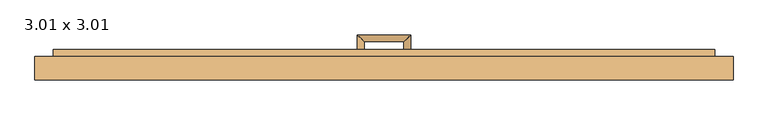
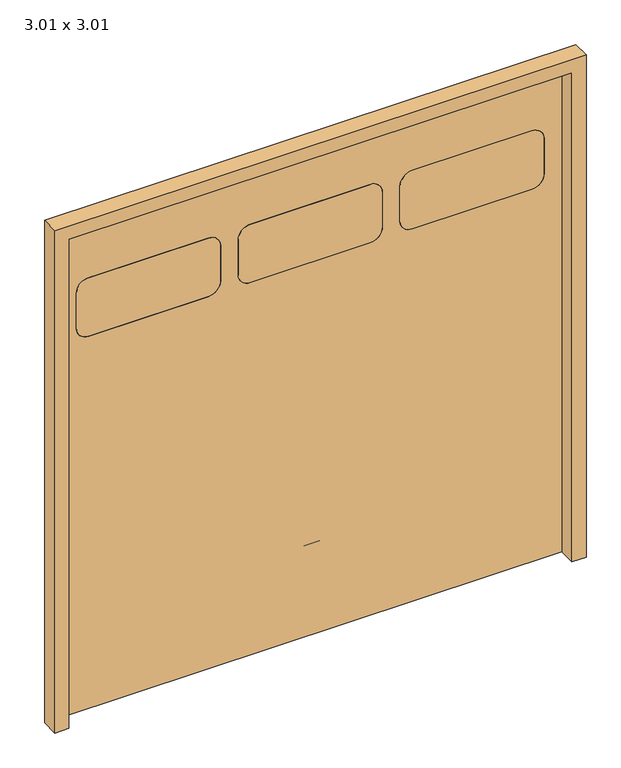
"""IFC4 building model written with IfcOpenShell, lengths in millimetres: door geometry, Garagentor : 3.01 x 3.01."""

from ifc_helpers import new_model, si_unit, point, frame, frame_2d, origin, place, context, project, spatial, polyline, circle_curve, ellipse_curve, trimmed, segment, composite_curve, outline, extrude, source, transform, mapped, element, save
from ifc_brep_helpers import plane_surface, cylinder_surface, advanced_brep


def door_3_01_x_3_01_f5100d20(model_context):
    return source(origin(), model_context, "Body", "SolidModel", [
        extrude(outline(composite_curve([segment(polyline([(2580.0, 1255.0), (2580.0, 578.3333333)]), True, "CONTINUOUS"), segment(trimmed(circle_curve(frame_2d((2510.0, 578.3333333)), 70.0), [point((2580.0, 578.3333333))], [point((2510.0, 508.3333333))], False, "CARTESIAN"), True, "CONTINUOUS"), segment(polyline([(2510.0, 508.3333333), (2300.0, 508.3333333)]), True, "CONTINUOUS"), segment(trimmed(circle_curve(frame_2d((2300.0, 578.3333333)), 70.0), [point((2300.0, 508.3333333))], [point((2230.0, 578.3333333))], False, "CARTESIAN"), True, "CONTINUOUS"), segment(polyline([(2230.0, 578.3333333), (2230.0, 1255.0)]), True, "CONTINUOUS"), segment(trimmed(circle_curve(frame_2d((2300.0, 1255.0)), 70.0), [point((2230.0, 1255.0))], [point((2300.0, 1325.0))], False, "CARTESIAN"), True, "CONTINUOUS"), segment(polyline([(2300.0, 1325.0), (2510.0, 1325.0)]), True, "CONTINUOUS"), segment(trimmed(circle_curve(frame_2d((2510.0, 1255.0)), 70.0), [point((2510.0, 1325.0))], [point((2580.0, 1255.0))], False, "CARTESIAN"), True, "CONTINUOUS")], self_intersect=False)), frame((0.0, -138.4216391, 0.0), z_axis=(0.0, 1.0, 0.0), x_axis=(0.0, 0.0, 1.0)), (0.0, 0.0, 1.0), 30.0),
        extrude(outline(composite_curve([segment(trimmed(circle_curve(frame_2d((2510.0, 338.3333333)), 70.0), [point((2510.0, 408.3333333))], [point((2580.0, 338.3333333))], False, "CARTESIAN"), True, "CONTINUOUS"), segment(polyline([(2580.0, 338.3333333), (2580.0, -338.3333333)]), True, "CONTINUOUS"), segment(trimmed(circle_curve(frame_2d((2510.0, -338.3333333)), 70.0), [point((2580.0, -338.3333333))], [point((2510.0, -408.3333333))], False, "CARTESIAN"), True, "CONTINUOUS"), segment(polyline([(2510.0, -408.3333333), (2300.0, -408.3333333)]), True, "CONTINUOUS"), segment(trimmed(circle_curve(frame_2d((2300.0, -338.3333333)), 70.0), [point((2300.0, -408.3333333))], [point((2230.0, -338.3333333))], False, "CARTESIAN"), True, "CONTINUOUS"), segment(polyline([(2230.0, -338.3333333), (2230.0, 338.3333333)]), True, "CONTINUOUS"), segment(trimmed(circle_curve(frame_2d((2300.0, 338.3333333)), 70.0), [point((2230.0, 338.3333333))], [point((2300.0, 408.3333333))], False, "CARTESIAN"), True, "CONTINUOUS"), segment(polyline([(2300.0, 408.3333333), (2510.0, 408.3333333)]), True, "CONTINUOUS")], self_intersect=False)), frame((0.0, -138.4216391, 0.0), z_axis=(0.0, 1.0, 0.0), x_axis=(0.0, 0.0, 1.0)), (0.0, 0.0, 1.0), 30.0),
        extrude(outline(composite_curve([segment(trimmed(circle_curve(frame_2d((2510.0, -578.3333333)), 70.0), [point((2510.0, -508.3333333))], [point((2580.0, -578.3333333))], False, "CARTESIAN"), True, "CONTINUOUS"), segment(polyline([(2580.0, -578.3333333), (2580.0, -1255.0)]), True, "CONTINUOUS"), segment(trimmed(circle_curve(frame_2d((2510.0, -1255.0)), 70.0), [point((2580.0, -1255.0))], [point((2510.0, -1325.0))], False, "CARTESIAN"), True, "CONTINUOUS"), segment(polyline([(2510.0, -1325.0), (2300.0, -1325.0)]), True, "CONTINUOUS"), segment(trimmed(circle_curve(frame_2d((2300.0, -1255.0)), 70.0), [point((2300.0, -1325.0))], [point((2230.0, -1255.0))], False, "CARTESIAN"), True, "CONTINUOUS"), segment(polyline([(2230.0, -1255.0), (2230.0, -578.3333333)]), True, "CONTINUOUS"), segment(trimmed(circle_curve(frame_2d((2300.0, -578.3333333)), 70.0), [point((2230.0, -578.3333333))], [point((2300.0, -508.3333333))], False, "CARTESIAN"), True, "CONTINUOUS"), segment(polyline([(2300.0, -508.3333333), (2510.0, -508.3333333)]), True, "CONTINUOUS")], self_intersect=False)), frame((0.0, -138.4216391, 0.0), z_axis=(0.0, 1.0, 0.0), x_axis=(0.0, 0.0, 1.0)), (0.0, 0.0, 1.0), 30.0),
        extrude(outline(polyline([(0.0, -1425.0), (0.0, 1425.0), (2930.0, 1425.0), (2930.0, -1425.0), (0.0, -1425.0)]), holes=[composite_curve([segment(polyline([(2580.0, 578.3333333), (2580.0, 1255.0)]), True, "CONTINUOUS"), segment(trimmed(circle_curve(frame_2d((2510.0, 1255.0)), 70.0), [point((2580.0, 1255.0))], [point((2510.0, 1325.0))], True, "CARTESIAN"), True, "CONTINUOUS"), segment(polyline([(2510.0, 1325.0), (2300.0, 1325.0)]), True, "CONTINUOUS"), segment(trimmed(circle_curve(frame_2d((2300.0, 1255.0)), 70.0), [point((2300.0, 1325.0))], [point((2230.0, 1255.0))], True, "CARTESIAN"), True, "CONTINUOUS"), segment(polyline([(2230.0, 1255.0), (2230.0, 578.3333333)]), True, "CONTINUOUS"), segment(trimmed(circle_curve(frame_2d((2300.0, 578.3333333)), 70.0), [point((2230.0, 578.3333333))], [point((2300.0, 508.3333333))], True, "CARTESIAN"), True, "CONTINUOUS"), segment(polyline([(2300.0, 508.3333333), (2510.0, 508.3333333)]), True, "CONTINUOUS"), segment(trimmed(circle_curve(frame_2d((2510.0, 578.3333333)), 70.0), [point((2510.0, 508.3333333))], [point((2580.0, 578.3333333))], True, "CARTESIAN"), True, "CONTINUOUS")], self_intersect=False), composite_curve([segment(polyline([(2580.0, -338.3333333), (2580.0, 338.3333333)]), True, "CONTINUOUS"), segment(trimmed(circle_curve(frame_2d((2510.0, 338.3333333)), 70.0), [point((2580.0, 338.3333333))], [point((2510.0, 408.3333333))], True, "CARTESIAN"), True, "CONTINUOUS"), segment(polyline([(2510.0, 408.3333333), (2300.0, 408.3333333)]), True, "CONTINUOUS"), segment(trimmed(circle_curve(frame_2d((2300.0, 338.3333333)), 70.0), [point((2300.0, 408.3333333))], [point((2230.0, 338.3333333))], True, "CARTESIAN"), True, "CONTINUOUS"), segment(polyline([(2230.0, 338.3333333), (2230.0, -338.3333333)]), True, "CONTINUOUS"), segment(trimmed(circle_curve(frame_2d((2300.0, -338.3333333)), 70.0), [point((2230.0, -338.3333333))], [point((2300.0, -408.3333333))], True, "CARTESIAN"), True, "CONTINUOUS"), segment(polyline([(2300.0, -408.3333333), (2510.0, -408.3333333)]), True, "CONTINUOUS"), segment(trimmed(circle_curve(frame_2d((2510.0, -338.3333333)), 70.0), [point((2510.0, -408.3333333))], [point((2580.0, -338.3333333))], True, "CARTESIAN"), True, "CONTINUOUS")], self_intersect=False), composite_curve([segment(polyline([(2580.0, -1255.0), (2580.0, -578.3333333)]), True, "CONTINUOUS"), segment(trimmed(circle_curve(frame_2d((2510.0, -578.3333333)), 70.0), [point((2580.0, -578.3333333))], [point((2510.0, -508.3333333))], True, "CARTESIAN"), True, "CONTINUOUS"), segment(polyline([(2510.0, -508.3333333), (2300.0, -508.3333333)]), True, "CONTINUOUS"), segment(trimmed(circle_curve(frame_2d((2300.0, -578.3333333)), 70.0), [point((2300.0, -508.3333333))], [point((2230.0, -578.3333333))], True, "CARTESIAN"), True, "CONTINUOUS"), segment(polyline([(2230.0, -578.3333333), (2230.0, -1255.0)]), True, "CONTINUOUS"), segment(trimmed(circle_curve(frame_2d((2300.0, -1255.0)), 70.0), [point((2230.0, -1255.0))], [point((2300.0, -1325.0))], True, "CARTESIAN"), True, "CONTINUOUS"), segment(polyline([(2300.0, -1325.0), (2510.0, -1325.0)]), True, "CONTINUOUS"), segment(trimmed(circle_curve(frame_2d((2510.0, -1255.0)), 70.0), [point((2510.0, -1325.0))], [point((2580.0, -1255.0))], True, "CARTESIAN"), True, "CONTINUOUS")], self_intersect=False)]), frame((0.0, -138.4216391, 0.0), z_axis=(0.0, 1.0, 0.0), x_axis=(0.0, 0.0, 1.0)), (0.0, 0.0, 1.0), 30.0),
        advanced_brep(
        [(-85.0, -108.4216391, 500.0), (-115.0, -108.4216391, 500.0), (-85.0, -73.4216391, 500.0), (-115.0, -43.4216391, 500.0), (85.0, -73.4216391, 500.0), (115.0, -43.4216391, 500.0), (85.0, -108.4216391, 500.0), (115.0, -108.4216391, 500.0)],
        [
            (0, 1, circle_curve(frame((-100.0, -108.4216391, 500.0), z_axis=(0.0, -1.0, 0.0), x_axis=(-1.0, 0.0, 0.0)), 15.0)),
            (1, 0, circle_curve(frame((-100.0, -108.4216391, 500.0), z_axis=(0.0, -1.0, 0.0), x_axis=(-1.0, 0.0, 0.0)), 15.0)),
            (0, 2),
            (2, 3, ellipse_curve(frame((-100.0, -58.4216391, 500.0), z_axis=(-0.7071067811865464, -0.7071067811865487, 0.0), x_axis=(0.7071067811865487, -0.7071067811865464, 0.0)), 21.2132034, 15.0)),
            (3, 1),
            (3, 2, ellipse_curve(frame((-100.0, -58.4216391, 500.0), z_axis=(-0.7071067811865464, -0.7071067811865487, 0.0), x_axis=(0.7071067811865487, -0.7071067811865464, 0.0)), 21.2132034, 15.0)),
            (2, 4),
            (4, 5, ellipse_curve(frame((100.0, -58.4216391, 500.0), z_axis=(-0.70710678118655, 0.7071067811865451, 0.0), x_axis=(-0.7071067811865449, -0.7071067811865501, 0.0)), 21.2132034, 15.0)),
            (5, 3),
            (5, 4, ellipse_curve(frame((100.0, -58.4216391, 500.0), z_axis=(-0.70710678118655, 0.7071067811865451, 0.0), x_axis=(-0.7071067811865449, -0.7071067811865501, 0.0)), 21.2132034, 15.0)),
            (6, 7, circle_curve(frame((100.0, -108.4216391, 500.0), z_axis=(0.0, -1.0, 0.0), x_axis=(1.0, 0.0, 0.0)), 15.0)),
            (7, 6, circle_curve(frame((100.0, -108.4216391, 500.0), z_axis=(0.0, -1.0, 0.0), x_axis=(1.0, 0.0, 0.0)), 15.0)),
            (4, 6),
            (7, 5),
        ],
        [
            plane_surface(frame((-100.0, -108.4216391, 500.0), z_axis=(0.0, -1.0, 0.0), x_axis=(0.0, 0.0, 1.0))),
            cylinder_surface(frame((-100.0, -108.4216391, 500.0), z_axis=(0.0, -1.0, 0.0), x_axis=(-1.0, 0.0, 0.0)), 15.0),
            cylinder_surface(frame((-100.0, -58.4216391, 500.0), z_axis=(-1.0, 0.0, 0.0), x_axis=(0.0, 1.0, 0.0)), 15.0),
            plane_surface(frame((100.0, -108.4216391, 500.0), z_axis=(0.0, -1.0, 0.0), x_axis=(0.0, 0.0, 1.0))),
            cylinder_surface(frame((100.0, -58.4216391, 500.0), z_axis=(0.0, 1.0, 0.0), x_axis=(1.0, 0.0, 0.0)), 15.0),
        ],
        [
            (0, [[1, 2]]),
            (1, [[-1, 3, 4, 5]]),
            (1, [[-2, -5, 6, -3]]),
            (2, [[-4, 7, 8, 9]]),
            (2, [[-6, -9, 10, -7]]),
            (3, [[11, 12]]),
            (4, [[-8, 13, -12, 14]]),
            (4, [[-10, -14, -11, -13]]),
        ],
    ),
        extrude(outline(polyline([(0.0, 1425.0), (0.0, 1505.0), (3010.0, 1505.0), (3010.0, -1505.0), (0.0, -1505.0), (0.0, -1425.0), (2930.0, -1425.0), (2930.0, 1425.0), (0.0, 1425.0)])), frame((0.0, -238.4216391, 0.0), z_axis=(0.0, 1.0, 0.0), x_axis=(0.0, 0.0, 1.0)), (0.0, 0.0, 1.0), 100.0),
    ])


if __name__ == "__main__":
    model = new_model("IFC4")
    model_context = context("Model", 3, world=origin())
    ifc_project = project(units=[si_unit("LENGTHUNIT", "METRE", prefix="MILLI")], contexts=[model_context])
    site = spatial("IfcSite", under=ifc_project)
    building = spatial("IfcBuilding", under=site)
    placement = place(None, origin())
    door_3_01_x_3_01_shape = door_3_01_x_3_01_f5100d20(model_context)
    element("IfcDoor", 1, ObjectType="Garagentor : 3.01 x 3.01", at=placement, inside=building, context=model_context, shape_type="MappedRepresentation", body=[
        mapped(door_3_01_x_3_01_shape, transform((0.0, 0.0, 0.0), x_axis=(1.0, 0.0, 0.0), y_axis=(0.0, 1.0, 0.0), z_axis=(0.0, 0.0, 1.0))),
    ])
    save(model, "model.ifc")

# Revit data of these elements
# Type "Garagentor : 3.01 x 3.01"
#   Type Mark = "21"
#   Operation = "RollingUp"
#   Keynote = "16.03"
#   Heat Transfer Coefficient (U) = 3.7021 W/(m²·K)
#   Rough Width = 3.010 m
#   Rahmentiefe = 0.100 m
#   Rahmenhöhe - oben = 0.100 m
#   Rahmenbreite = 0.080 m
#   Rough Height [instance default] = 3.110 m
#   Höhe Füllung = 2.930 m
#   Breite Füllung = 2.850 m
#   Height = 3.010 m
#   Fußbodenaufbau [instance default] = 0.100 m
#   Einbautiefe (von außen) [instance default] = 0.050 m
#   Width = 3.010 m
#   Sichtbarkeit Sturzlinien [instance default] = yes
#   Function = 1
#   Glas [instance default] = none
#   Tor [instance default] = none
#   Rahmen/Pfosten [instance default] = none
#   Füllung [instance default] = element 471010
#   Visual Light Transmittance = 0
#   Solar Heat Gain Coefficient = 0
#   Construction Type Id = ""
#   Wall Closure = (empty or 0)
#   Analytic Construction = (empty or 0)
# Element 1 (IfcDoor, "Garagentor : 3.01 x 3.01")
#   Rough Height = 3.010 m
#   Fußbodenaufbau = 0.000 m
#   Einbautiefe (von außen) = 0.000 m
#   Materials on its faces: "Holz - Birke", "Glas", "Metall - Chrom"
# Materials
#   "Holz - Birke": class "Holz", colour RGB 213 164 103, transparency 0, Cost = 0
#   "Glas": class "Glas", colour RGB 0 0 255, transparency 0.75, Comments = "Render-Darstellung nicht aktualisiert ", Cost = 0
#   "Metall - Chrom": class "Metall", colour RGB 247 247 247, transparency 0, Cost = 0
